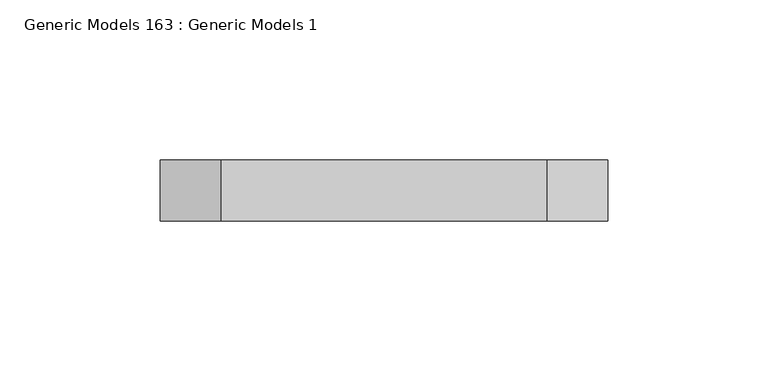
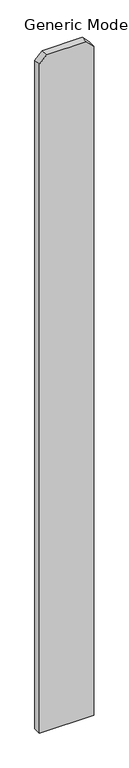
"""IFC4 building model written with IfcOpenShell, lengths in millimetres: proxy geometry, Generic Models 163 : Generic Models 1."""

from ifc_helpers import new_model, si_unit, frame, origin, place, context, project, spatial, polyline, outline, extrude, source, transform, mapped, element, save


def generic_models_163_generic_models_1_49017f73(model_context):
    return source(origin(), model_context, "Body", "SweptSolid", [
        extrude(outline(polyline([(76.2, -249962.9875), (1885.95, -249962.9875), (1905.0, -249982.0375), (1905.0, -250083.6375), (1885.95, -250102.6875), (76.2, -250102.6875), (76.2, -249962.9875)])), frame((0.0, 547.6875, 0.0), z_axis=(0.0, 1.0, 0.0), x_axis=(0.0, 0.0, 1.0)), (0.0, 0.0, 1.0), 19.05),
    ])


if __name__ == "__main__":
    model = new_model("IFC4")
    model_context = context("Model", 3, world=origin())
    ifc_project = project(units=[si_unit("LENGTHUNIT", "METRE", prefix="MILLI")], contexts=[model_context])
    site = spatial("IfcSite", under=ifc_project)
    building = spatial("IfcBuilding", under=site)
    placement = place(None, origin())
    generic_models_163_generic_models_1_shape = generic_models_163_generic_models_1_49017f73(model_context)
    element("IfcBuildingElementProxy", 1, Name="Generic Models 163 : Generic Models 1", ObjectType="Generic Models 163 : Generic Models 1", at=placement, inside=building, context=model_context, shape_type="MappedRepresentation", body=[
        mapped(generic_models_163_generic_models_1_shape, transform((0.0, 0.0, 0.0), x_axis=(1.0, 0.0, 0.0), y_axis=(0.0, 1.0, 0.0), z_axis=(0.0, 0.0, 1.0))),
    ])
    save(model, "model.ifc")

# Revit data of these elements
# Element 1 (IfcBuildingElementProxy, "Generic Models 163 : Generic Models 1")
#   Materials on its faces: "VERTICAL 1X6 CEDAR PLANKS W/ CLEAR WOOD SEALER"
# Materials
#   "VERTICAL 1X6 CEDAR PLANKS W/ CLEAR WOOD SEALER": class "Wood", colour RGB 234 198 147, transparency 0, Description = "Pinus Echinata", Cost = 0
